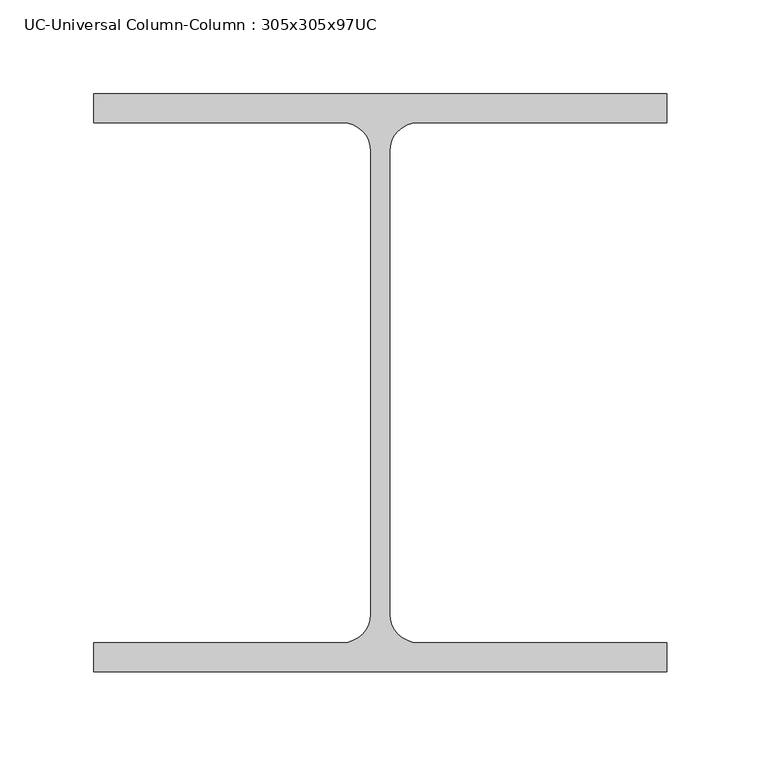
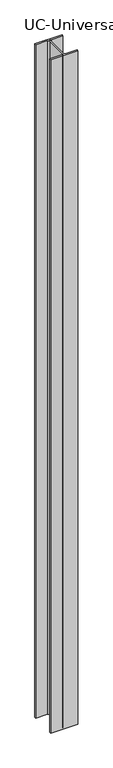
"""IFC4 building model written with IfcOpenShell, lengths in millimetres: column geometry, UC-Universal Column-Column : 305x305x97UC."""

from ifc_helpers import new_model, si_unit, point, frame_2d, origin, origin_with_axes, place, context, project, spatial, polyline, circle_curve, trimmed, segment, composite_curve, outline, extrude, source, transform, mapped, element, save


def uc_universal_column_column_305x305x97uc_b32ae94d(model_context):
    return source(origin(), model_context, "Body", "SweptSolid", [
        extrude(outline(composite_curve([segment(polyline([(152.65, 153.95), (152.65, 138.55), (20.15, 138.55)]), True, "CONTINUOUS"), segment(trimmed(circle_curve(frame_2d((20.15, 123.35)), 15.2), [point((20.15, 138.55))], [point((4.95, 123.35))], True, "CARTESIAN"), True, "CONTINUOUS"), segment(polyline([(4.95, 123.35), (4.95, -123.35)]), True, "CONTINUOUS"), segment(trimmed(circle_curve(frame_2d((20.15, -123.35)), 15.2), [point((4.95, -123.35))], [point((20.15, -138.55))], True, "CARTESIAN"), True, "CONTINUOUS"), segment(polyline([(20.15, -138.55), (152.65, -138.55), (152.65, -153.95), (-152.65, -153.95), (-152.65, -138.55), (-20.15, -138.55)]), True, "CONTINUOUS"), segment(trimmed(circle_curve(frame_2d((-20.15, -123.35)), 15.2), [point((-20.15, -138.55))], [point((-4.95, -123.35))], True, "CARTESIAN"), True, "CONTINUOUS"), segment(polyline([(-4.95, -123.35), (-4.95, 123.35)]), True, "CONTINUOUS"), segment(trimmed(circle_curve(frame_2d((-20.15, 123.35)), 15.2), [point((-4.95, 123.35))], [point((-20.15, 138.55))], True, "CARTESIAN"), True, "CONTINUOUS"), segment(polyline([(-20.15, 138.55), (-152.65, 138.55), (-152.65, 153.95), (152.65, 153.95)]), True, "CONTINUOUS")], self_intersect=False)), origin_with_axes(), (0.0, 0.0, 1.0), 8000.0),
    ])


if __name__ == "__main__":
    model = new_model("IFC4")
    model_context = context("Model", 3, world=origin())
    ifc_project = project(units=[si_unit("LENGTHUNIT", "METRE", prefix="MILLI")], contexts=[model_context])
    site = spatial("IfcSite", under=ifc_project)
    building = spatial("IfcBuilding", under=site)
    placement = place(None, origin())
    uc_universal_column_column_305x305x97uc_shape = uc_universal_column_column_305x305x97uc_b32ae94d(model_context)
    element("IfcColumn", 1, ObjectType="UC-Universal Column-Column : 305x305x97UC", at=placement, inside=building, context=model_context, shape_type="MappedRepresentation", body=[
        mapped(uc_universal_column_column_305x305x97uc_shape, transform((0.0, 0.0, 0.0), x_axis=(1.0, 0.0, 0.0), y_axis=(0.0, 1.0, 0.0), z_axis=(0.0, 0.0, 1.0))),
    ])
    save(model, "model.ifc")

# Revit data of these elements
# Type "UC-Universal Column-Column : 305x305x97UC"
#   Nominal h = "305"
#   W = 0
#   Ix = 22250
#   M = 96.9
#   Zx = 1445
#   b = 305.3 mm
#   h = 307.9 mm
#   r = 15.2 mm
#   s = 9.9 mm
#   t = 15.4 mm
#   A = 0.0123 m²
#   Structural Material [instance default] = Metal - Steel - 345 MPa
#   Assembly Code = ""
# Element 1 (IfcColumn, "UC-Universal Column-Column : 305x305x97UC")
#   Materials on its faces: "Metal - Steel - 345 MPa"
# Materials
#   "Metal - Steel - 345 MPa": class "Metal", colour RGB 241 46 46, transparency 0
